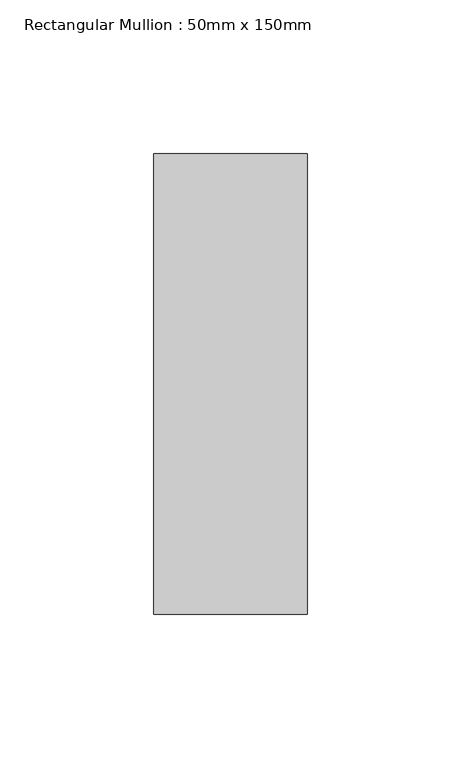
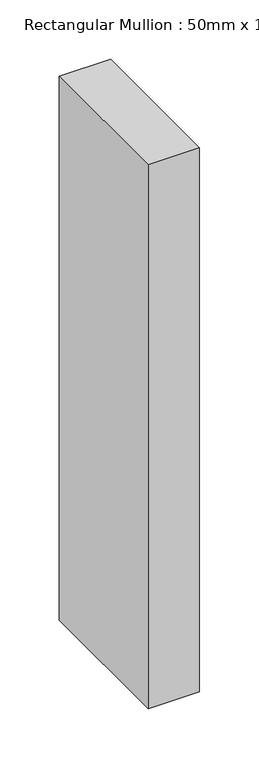
"""IFC4 building model written with IfcOpenShell, lengths in millimetres: member geometry, Rectangular Mullion : 50mm x 150mm."""

from ifc_helpers import new_model, si_unit, frame, origin, place, context, project, spatial, polyline, outline, extrude, source, transform, mapped, element, save


def rectangular_mullion_50mm_x_150mm_579c010a(model_context):
    return source(origin(), model_context, "Body", "SweptSolid", [
        extrude(outline(polyline([(0.0, 75.0), (0.0, -75.0), (-50.0, -75.0), (-50.0, 75.0), (0.0, 75.0)])), frame((0.0, 0.0, -560.51442), z_axis=(0.0, 0.0, 1.0), x_axis=(1.0, 0.0, 0.0)), (0.0, 0.0, 1.0), 560.51442),
    ])


if __name__ == "__main__":
    model = new_model("IFC4")
    model_context = context("Model", 3, world=origin())
    ifc_project = project(units=[si_unit("LENGTHUNIT", "METRE", prefix="MILLI")], contexts=[model_context])
    site = spatial("IfcSite", under=ifc_project)
    building = spatial("IfcBuilding", under=site)
    placement = place(None, origin())
    rectangular_mullion_50mm_x_150mm_shape = rectangular_mullion_50mm_x_150mm_579c010a(model_context)
    element("IfcMember", 1, ObjectType="Rectangular Mullion : 50mm x 150mm", at=placement, inside=building, context=model_context, shape_type="MappedRepresentation", body=[
        mapped(rectangular_mullion_50mm_x_150mm_shape, transform((0.0, 0.0, 0.0), x_axis=(1.0, 0.0, 0.0), y_axis=(0.0, 1.0, 0.0), z_axis=(0.0, 0.0, 1.0))),
    ])
    save(model, "model.ifc")

# Revit data of these elements
# Type "Rectangular Mullion : 50mm x 150mm"
#   built-in parameter 1007304 = 0.492126 (stored number, unit not read)
#   built-in parameter 1007301 = 0.082021 (stored number, unit not read)
#   built-in parameter 1007300 = 0.082021 (stored number, unit not read)
# Element 1 (IfcMember, "Rectangular Mullion : 50mm x 150mm")
#   Materials on its faces: "Aluminum"
# Materials
#   "Aluminum": class "Metal", colour RGB 247 247 247, transparency 0, Description = "Aluminum 6061", Cost = 0
